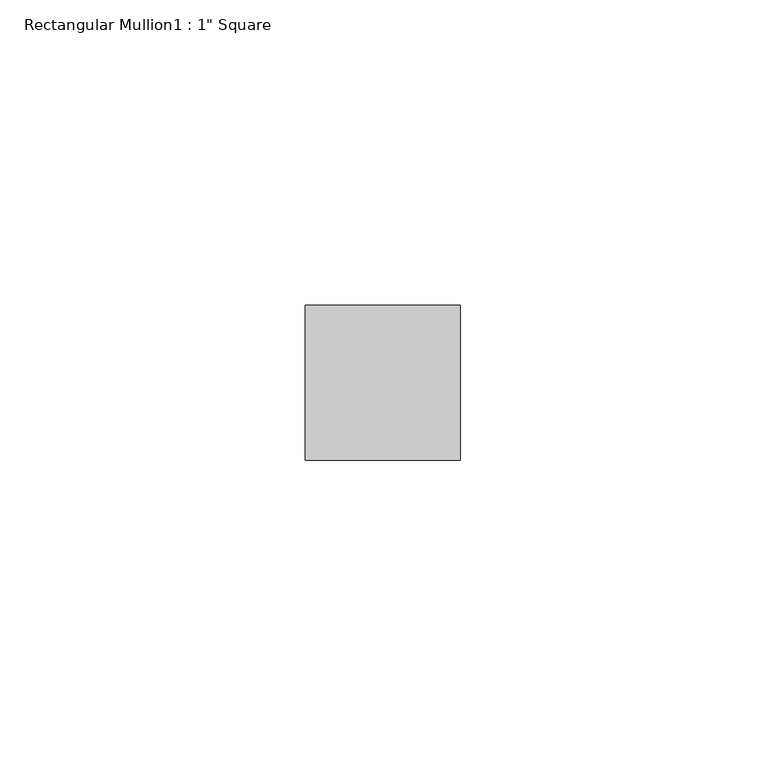
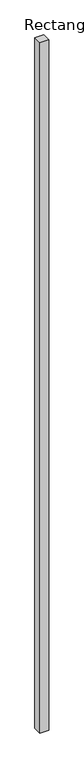
"""IFC4 building model written with IfcOpenShell, lengths in millimetres: member geometry."""

from ifc_helpers import new_model, si_unit, frame, origin, place, context, project, spatial, polyline, outline, extrude, source, transform, mapped, element, save


def member_99ddd2ca(model_context):
    return source(origin(), model_context, "Body", "SweptSolid", [
        extrude(outline(polyline([(12.7, -19.05), (12.7, -44.45), (-12.7, -44.45), (-12.7, -19.05), (12.7, -19.05)])), frame((0.0, 0.0, -2108.2), z_axis=(0.0, 0.0, 1.0), x_axis=(1.0, 0.0, 0.0)), (0.0, 0.0, 1.0), 2108.2),
    ])


if __name__ == "__main__":
    model = new_model("IFC4")
    model_context = context("Model", 3, world=origin())
    ifc_project = project(units=[si_unit("LENGTHUNIT", "METRE", prefix="MILLI")], contexts=[model_context])
    site = spatial("IfcSite", under=ifc_project)
    building = spatial("IfcBuilding", under=site)
    placement = place(None, origin())
    member_shape = member_99ddd2ca(model_context)
    element("IfcMember", 1, ObjectType="Rectangular Mullion1 : 1\" Square", at=placement, inside=building, context=model_context, shape_type="MappedRepresentation", body=[
        mapped(member_shape, transform((0.0, 0.0, 0.0), x_axis=(1.0, 0.0, 0.0), y_axis=(0.0, 1.0, 0.0), z_axis=(0.0, 0.0, 1.0))),
    ])
    save(model, "model.ifc")

# Revit data of these elements
# Type "Rectangular Mullion1 : 1\" Square"
#   built-in parameter 1007351 = 0.104167 (stored number, unit not read)
#   built-in parameter 1007304 = 0.0833333 (stored number, unit not read)
#   built-in parameter 1007301 = 0.0416667 (stored number, unit not read)
#   built-in parameter 1007300 = 0.0416667 (stored number, unit not read)
